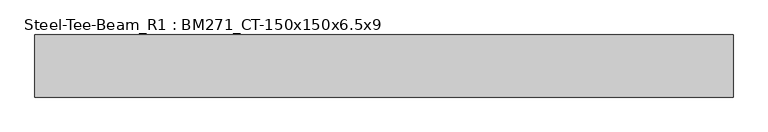
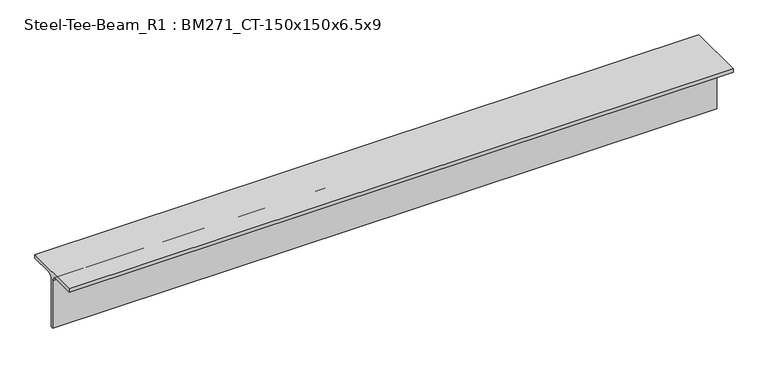
"""IFC4 building model written with IfcOpenShell, lengths in millimetres: member geometry, Steel-Tee-Beam_R1 : BM271_CT-150x150x6.5x9."""

from ifc_helpers import new_model, si_unit, point, frame, frame_2d, origin, place, context, project, spatial, polyline, circle_curve, trimmed, segment, composite_curve, outline, extrude, source, transform, mapped, element, save


def steel_tee_beam_r1_bm271_ct_150x150x6_5x9_8ea5b858(model_context):
    return source(origin(), model_context, "Body", "SweptSolid", [
        extrude(outline(composite_curve([segment(polyline([(75.0, 75.0), (75.0, 66.0), (16.25, 66.0)]), True, "CONTINUOUS"), segment(trimmed(circle_curve(frame_2d((16.25, 53.0)), 13.0), [point((16.25, 66.0))], [point((3.25, 53.0))], True, "CARTESIAN"), True, "CONTINUOUS"), segment(polyline([(3.25, 53.0), (3.25, -75.0), (-3.25, -75.0), (-3.25, 53.0)]), True, "CONTINUOUS"), segment(trimmed(circle_curve(frame_2d((-16.25, 53.0)), 13.0), [point((-3.25, 53.0))], [point((-16.25, 66.0))], True, "CARTESIAN"), True, "CONTINUOUS"), segment(polyline([(-16.25, 66.0), (-75.0, 66.0), (-75.0, 75.0), (75.0, 75.0)]), True, "CONTINUOUS")], self_intersect=False)), frame((-842.322898, 0.0, 0.0), z_axis=(1.0, 0.0, 0.0), x_axis=(0.0, 1.0, 0.0)), (0.0, 0.0, 1.0), 1684.6457959),
    ])


if __name__ == "__main__":
    model = new_model("IFC4")
    model_context = context("Model", 3, world=origin())
    ifc_project = project(units=[si_unit("LENGTHUNIT", "METRE", prefix="MILLI")], contexts=[model_context])
    site = spatial("IfcSite", under=ifc_project)
    building = spatial("IfcBuilding", under=site)
    placement = place(None, origin())
    steel_tee_beam_r1_bm271_ct_150x150x6_5x9_shape = steel_tee_beam_r1_bm271_ct_150x150x6_5x9_8ea5b858(model_context)
    element("IfcMember", 1, ObjectType="Steel-Tee-Beam_R1 : BM271_CT-150x150x6.5x9", at=placement, inside=building, context=model_context, shape_type="MappedRepresentation", body=[
        mapped(steel_tee_beam_r1_bm271_ct_150x150x6_5x9_shape, transform((0.0, 0.0, 0.0), x_axis=(1.0, 0.0, 0.0), y_axis=(0.0, 1.0, 0.0), z_axis=(0.0, 0.0, 1.0))),
    ])
    save(model, "model.ifc")

# Revit data of these elements
# Type "Steel-Tee-Beam_R1 : BM271_CT-150x150x6.5x9"
#   Keynote = "CT-150x150x6.5x9"
#   Surface Area = 0.588841 m²/m
#   Section Area = 23.3904 cm²
#   Mass per Unit Length = 18.3614 kg/m
#   Length [instance default] = 1.5240 m
#   bf = 0.1500 m
#   d = 0.1500 m
#   k = 0.0220 m
#   r = 0.0130 m
#   tf = 0.0090 m
#   tw = 0.0065 m
#   hec_material4 [instance default] = none
#   hec_material3 [instance default] = none
#   hec_material2 [instance default] = none
#   hec_material1 [instance default] = none
#   Structural Material [instance default] = Steel, 45-345
#   Assembly Code = ""
# Element 1 (IfcMember, "Steel-Tee-Beam_R1 : BM271_CT-150x150x6.5x9")
#   Structural Material = none
# Materials
#   "Steel, 45-345": class "Metal", colour RGB 189 187 185, transparency 0, Description = "Steel 345 MPa", Cost = 0
